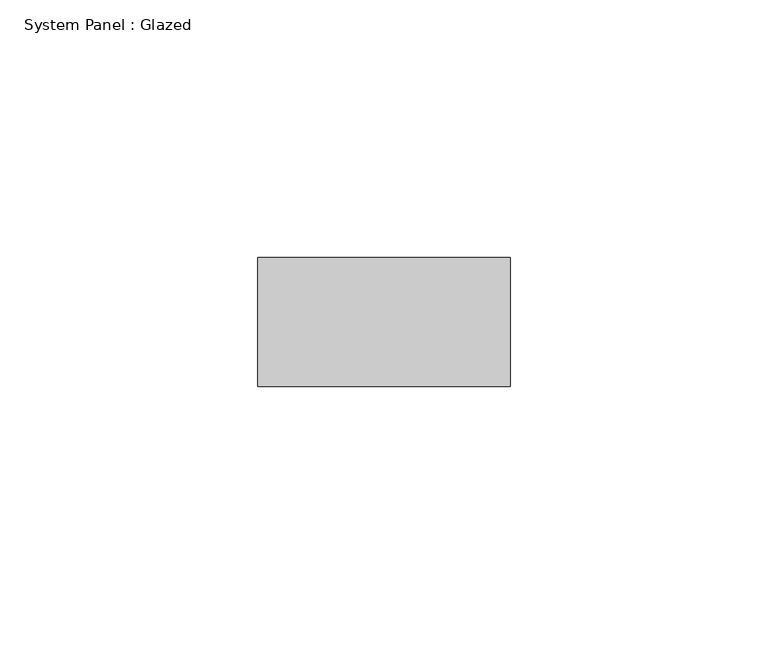
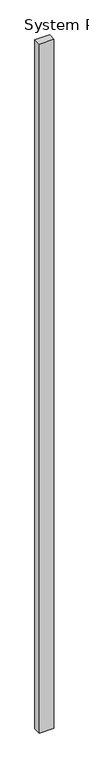
"""IFC4 building model written with IfcOpenShell, lengths in millimetres: plate geometry, System Panel : Glazed."""

from ifc_helpers import new_model, si_unit, origin, origin_with_axes, place, context, project, spatial, polyline, outline, extrude, source, transform, mapped, element, save


def system_panel_glazed_7067f38e(model_context):
    return source(origin(), model_context, "Body", "SweptSolid", [
        extrude(outline(polyline([(24.5092572, -49.5), (-24.5092572, -49.5), (-24.5092572, -24.5), (24.5092572, -24.5), (24.5092572, -49.5)])), origin_with_axes(), (0.0, 0.0, 1.0), 2425.0),
    ])


if __name__ == "__main__":
    model = new_model("IFC4")
    model_context = context("Model", 3, world=origin())
    ifc_project = project(units=[si_unit("LENGTHUNIT", "METRE", prefix="MILLI")], contexts=[model_context])
    site = spatial("IfcSite", under=ifc_project)
    building = spatial("IfcBuilding", under=site)
    placement = place(None, origin())
    system_panel_glazed_shape = system_panel_glazed_7067f38e(model_context)
    element("IfcPlate", 1, ObjectType="System Panel : Glazed", at=placement, inside=building, context=model_context, shape_type="MappedRepresentation", body=[
        mapped(system_panel_glazed_shape, transform((0.0, 0.0, 0.0), x_axis=(1.0, 0.0, 0.0), y_axis=(0.0, 1.0, 0.0), z_axis=(0.0, 0.0, 1.0))),
    ])
    save(model, "model.ifc")

# Revit data of these elements
# Type "System Panel : Glazed"
#   Keynote = "H11"
#   Construction Type Id = "GSP4R"
#   Analytic Construction = "1/8 in Pilkington single glazing"
#   Visual Light Transmittance = 0.9
#   Solar Heat Gain Coefficient = 0.86
#   Heat Transfer Coefficient (U) = 6.7069 W/(m²·K)
# Element 1 (IfcPlate, "System Panel : Glazed")
#   Materials on its faces: "Glass"
# Materials
#   "Glass": class "Glass", colour RGB 0 128 192, transparency 0.9, Description = "Soda Lime Glass", Cost = 0
